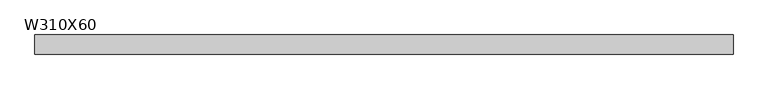
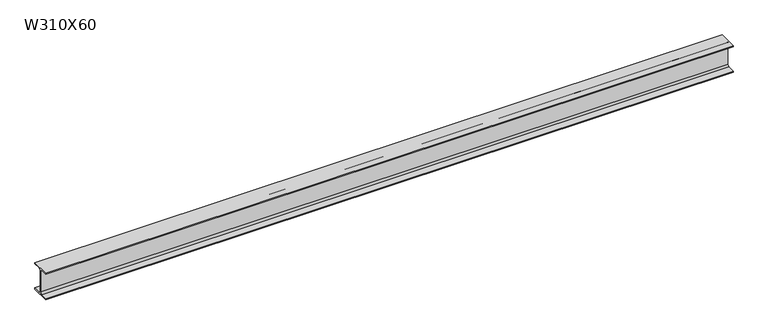
"""IFC4 building model written with IfcOpenShell, lengths in millimetres: beam geometry, M_W-Wide Flange : W310X60."""

from ifc_helpers import new_model, si_unit, point, frame, frame_2d, origin, place, context, project, spatial, polyline, circle_curve, trimmed, segment, composite_curve, outline, extrude, source, transform, mapped, element, save


def w310x60_0f32da04(model_context):
    return source(origin(), model_context, "Body", "SweptSolid", [
        extrude(outline(composite_curve([segment(polyline([(101.5, -138.4), (101.5, -151.5), (-101.5, -151.5), (-101.5, -138.4), (-23.65, -138.4)]), True, "CONTINUOUS"), segment(trimmed(circle_curve(frame_2d((-23.65, -118.5)), 19.9), [point((-23.65, -138.4))], [point((-3.75, -118.5))], True, "CARTESIAN"), True, "CONTINUOUS"), segment(polyline([(-3.75, -118.5), (-3.75, 118.5)]), True, "CONTINUOUS"), segment(trimmed(circle_curve(frame_2d((-23.65, 118.5)), 19.9), [point((-3.75, 118.5))], [point((-23.65, 138.4))], True, "CARTESIAN"), True, "CONTINUOUS"), segment(polyline([(-23.65, 138.4), (-101.5, 138.4), (-101.5, 151.5), (101.5, 151.5), (101.5, 138.4), (23.65, 138.4)]), True, "CONTINUOUS"), segment(trimmed(circle_curve(frame_2d((23.65, 118.5)), 19.9), [point((23.65, 138.4))], [point((3.75, 118.5))], True, "CARTESIAN"), True, "CONTINUOUS"), segment(polyline([(3.75, 118.5), (3.75, -118.5)]), True, "CONTINUOUS"), segment(trimmed(circle_curve(frame_2d((23.65, -118.5)), 19.9), [point((3.75, -118.5))], [point((23.65, -138.4))], True, "CARTESIAN"), True, "CONTINUOUS"), segment(polyline([(23.65, -138.4), (101.5, -138.4)]), True, "CONTINUOUS")], self_intersect=False)), frame((-3761.5, 0.0, 0.0), z_axis=(1.0, 0.0, 0.0), x_axis=(0.0, 1.0, 0.0)), (0.0, 0.0, 1.0), 7421.3),
    ])


if __name__ == "__main__":
    model = new_model("IFC4")
    model_context = context("Model", 3, world=origin())
    ifc_project = project(units=[si_unit("LENGTHUNIT", "METRE", prefix="MILLI")], contexts=[model_context])
    site = spatial("IfcSite", under=ifc_project)
    building = spatial("IfcBuilding", under=site)
    placement = place(None, origin())
    w310x60_shape = w310x60_0f32da04(model_context)
    element("IfcBeam", 1, ObjectType="M_W-Wide Flange : W310X60", at=placement, inside=building, context=model_context, shape_type="MappedRepresentation", body=[
        mapped(w310x60_shape, transform((0.0, 0.0, 0.0), x_axis=(1.0, 0.0, 0.0), y_axis=(0.0, 1.0, 0.0), z_axis=(0.0, 0.0, 1.0))),
    ])
    save(model, "model.ifc")

# Revit data of these elements
# Type "M_W-Wide Flange : W310X60"
#   Manufacturer = "Manufacturer"
#   AccessibilityPerformance = "AccessibilityPerformance"
#   CodePerformance = "CodePerformance"
#   Color = "Color"
#   Constituents = "Constituents"
#   Features = "Features"
#   Finish = "Finish"
#   Grade = "Grade"
#   Material = "Material"
#   ModelReference = "ModelReference"
#   NominalHeight = "NominalHeight"
#   NominalLength = "NominalLength"
#   NominalWidth = "NominalWidth"
#   ProductionYear = "ProductionYear"
#   Reference = "Reference"
#   Shape = "Shape"
#   Size = "Size"
#   SustainabilityPerformance = "SustainabilityPerformance"
#   WarrantyDescription = "WarrantyDescription"
#   WarrantyDurationLabor = "WarrantyDurationLabor"
#   WarrantyDurationParts = "WarrantyDurationParts"
#   WarrantyGuarantorLabor = "WarrantyGuarantorLabor"
#   WarrantyGuarantorParts = "WarrantyGuarantorParts"
#   ExpectedLife = "ExpectedLife"
#   ReplacementCost = "ReplacementCost"
#   AssetAccountingType = "FIXED"
#   ModelLabel = "ModelLabel"
#   W = 0.58
#   Start Extension Calculation [instance default] = 3.000 m
#   Start Extension [instance default] = -0.0127 m
#   End Extension Calculation [instance default] = 3.000 m
#   End Extension [instance default] = -0.0127 m
#   Length [instance default] = 1.524 m
#   bf = 0.203 m
#   d = 0.303 m
#   k = 0.033 m
#   kr = 0.0199 m
#   tf = 0.0131 m
#   tw = 0.0075 m
#   A = 0.00753 m²
#   Structural Material [instance default] = Metal - Steel - 345 MPa
#   Assembly Code = ""
# Element 1 (IfcBeam, "M_W-Wide Flange : W310X60")
#   Materials on its faces: "Metal - Steel - 345 MPa"
# Materials
#   "Metal - Steel - 345 MPa": class "Metal", colour RGB 247 247 247, transparency 0
